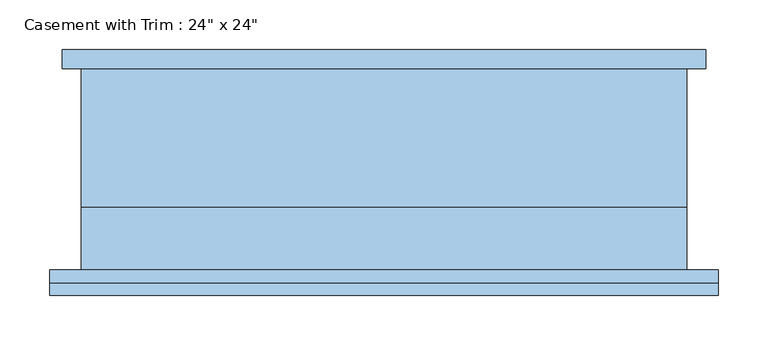
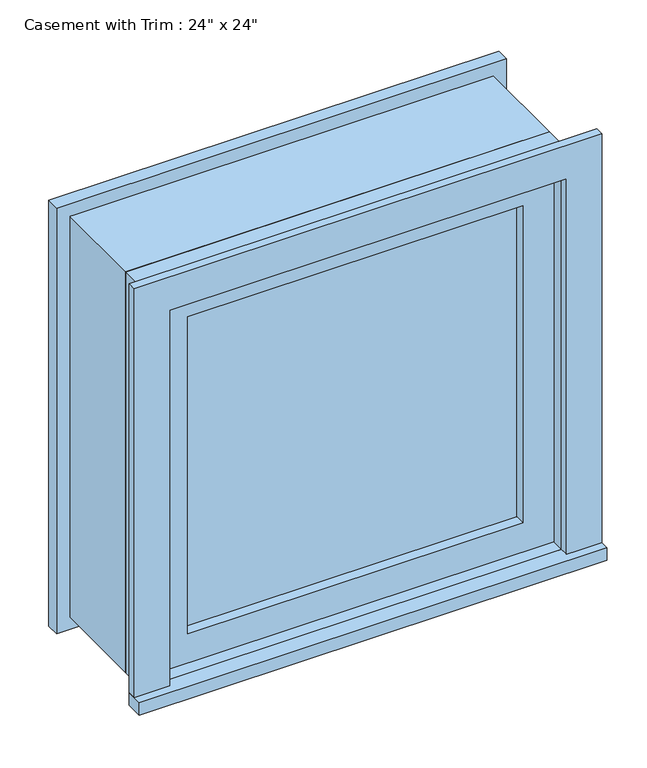
"""IFC4 building model written with IfcOpenShell, lengths in millimetres: window geometry."""

from ifc_helpers import new_model, si_unit, frame, origin, place, context, project, spatial, polyline, outline, extrude, source, transform, mapped, element, save


def window_fcd5a920(model_context):
    return source(origin(), model_context, "Body", "SweptSolid", [
        extrude(outline(polyline([(-336.55, -127.0), (-336.55, -101.6), (336.55, -101.6), (336.55, -127.0), (-336.55, -127.0)])), frame((0.0, 0.0, 914.4), z_axis=(0.0, 0.0, 1.0), x_axis=(1.0, 0.0, 0.0)), (0.0, 0.0, 1.0), 19.05),
        extrude(outline(polyline([(1504.95, -285.75), (1504.95, 285.75), (933.45, 285.75), (933.45, 336.55), (1555.75, 336.55), (1555.75, -336.55), (933.45, -336.55), (933.45, -285.75), (1504.95, -285.75)])), frame((0.0, -114.3, 0.0), z_axis=(0.0, 1.0, 0.0), x_axis=(0.0, 0.0, 1.0)), (0.0, 0.0, 1.0), 12.7),
        extrude(outline(polyline([(1543.05, 323.85), (1543.05, -323.85), (895.35, -323.85), (895.35, 323.85), (1543.05, 323.85)]), holes=[polyline([(1492.25, 273.05), (946.15, 273.05), (946.15, -273.05), (1492.25, -273.05), (1492.25, 273.05)])]), frame((0.0, 101.6, 0.0), z_axis=(0.0, 1.0, 0.0), x_axis=(0.0, 0.0, 1.0)), (0.0, 0.0, 1.0), 19.05),
        extrude(outline(polyline([(241.3, -53.975), (241.3, -66.675), (-241.3, -66.675), (-241.3, -53.975), (241.3, -53.975)])), frame((0.0, 0.0, 977.9), z_axis=(0.0, 0.0, 1.0), x_axis=(1.0, 0.0, 0.0)), (0.0, 0.0, 1.0), 482.6),
        extrude(outline(polyline([(1504.95, -285.75), (933.45, -285.75), (933.45, 285.75), (1504.95, 285.75), (1504.95, -285.75)]), holes=[polyline([(1460.5, -241.3), (1460.5, 241.3), (977.9, 241.3), (977.9, -241.3), (1460.5, -241.3)])]), frame((0.0, -82.55, 0.0), z_axis=(0.0, 1.0, 0.0), x_axis=(0.0, 0.0, 1.0)), (0.0, 0.0, 1.0), 44.45),
        extrude(outline(polyline([(1524.0, -304.8), (914.4, -304.8), (914.4, 304.8), (1524.0, 304.8), (1524.0, -304.8)]), holes=[polyline([(1492.25, -273.05), (1492.25, 273.05), (946.15, 273.05), (946.15, -273.05), (1492.25, -273.05)])]), frame((0.0, -38.1, 0.0), z_axis=(0.0, 1.0, 0.0), x_axis=(0.0, 0.0, 1.0)), (0.0, 0.0, 1.0), 139.7),
        extrude(outline(polyline([(1524.0, 304.8), (1524.0, -304.8), (914.4, -304.8), (914.4, 304.8), (1524.0, 304.8)]), holes=[polyline([(1504.95, 285.75), (933.45, 285.75), (933.45, -285.75), (1504.95, -285.75), (1504.95, 285.75)])]), frame((0.0, -101.6, 0.0), z_axis=(0.0, 1.0, 0.0), x_axis=(0.0, 0.0, 1.0)), (0.0, 0.0, 1.0), 63.5),
    ])


if __name__ == "__main__":
    model = new_model("IFC4")
    model_context = context("Model", 3, world=origin())
    ifc_project = project(units=[si_unit("LENGTHUNIT", "METRE", prefix="MILLI")], contexts=[model_context])
    site = spatial("IfcSite", under=ifc_project)
    building = spatial("IfcBuilding", under=site)
    placement = place(None, origin())
    window_shape = window_fcd5a920(model_context)
    element("IfcWindow", 1, ObjectType="Casement with Trim : 24\" x 24\"", at=placement, inside=building, context=model_context, shape_type="MappedRepresentation", body=[
        mapped(window_shape, transform((0.0, 0.0, 0.0), x_axis=(1.0, 0.0, 0.0), y_axis=(0.0, 1.0, 0.0), z_axis=(0.0, 0.0, 1.0))),
    ])
    save(model, "model.ifc")

# Revit data of these elements
# Type "Casement with Trim : 24\" x 24\""
#   Type Mark = "13"
#   Assembly Code = "B2020100"
#   Height = 2' - 0"
#   Default Sill Height = 3' - 0"
#   Trim Projection - Ext. = 0' - 0 1/2"
#   Trim Projection - Int. = 0' - 0 3/4"
#   Trim Width - Exterior = 0' - 2"
#   Trim Width - Interior = 0' - 2"
#   Width = 2' - 0"
#   Window Inset = 0' - 0 3/4"
#   Glass Pane Material = Glass
#   Sash Material = Sash
#   Trim Exterior Material = Trim
#   Trim Interior Material = Trim
#   Wall Closure = (empty or 0)
# Element 1 (IfcWindow, "Casement with Trim : 24\" x 24\"")
#   Materials on its faces: "Sash", "Trim", "Glass"
# Materials
#   "Glass": class "Glass", colour RGB 0 128 192, transparency 0.75
#   "Sash": class "Wood", colour RGB 224 178 126, transparency 0
#   "Trim": class "Wood", colour RGB 224 178 126, transparency 0
